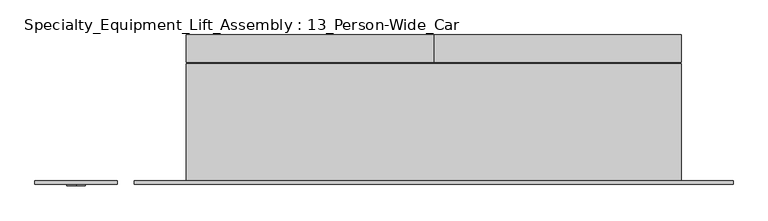
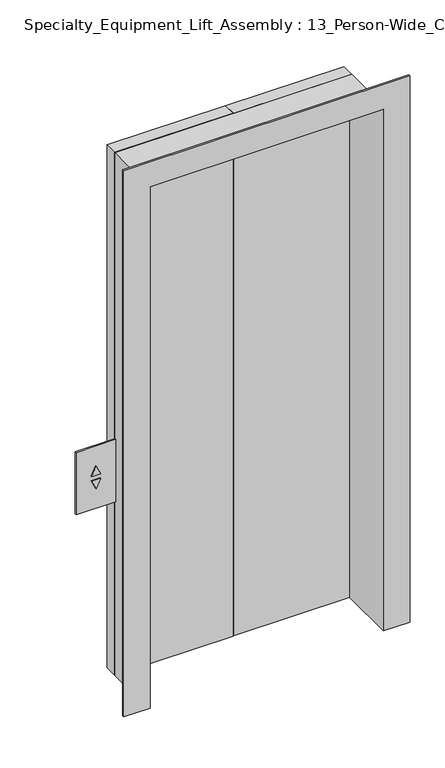
"""IFC4 building model written with IfcOpenShell, lengths in millimetres: proxy geometry, Specialty_Equipment_Lift_Assembly : 13_Person-Wide_Car."""

from ifc_helpers import new_model, si_unit, frame, origin, origin_with_axes, place, context, project, spatial, polyline, outline, extrude, faceted_brep, source, transform, mapped, element, save


def specialty_equipment_lift_assembly_13_person_wide_car_b1ef294d(model_context):
    return source(origin(), model_context, "Body", "SolidModel", [
        extrude(outline(polyline([(1008.7476885, -883.0952695), (1045.0, -900.0), (1008.7476885, -916.9047305), (1008.7476885, -883.0952695)])), frame((0.0, -116.5, 0.0), z_axis=(0.0, 1.0, 0.0), x_axis=(0.0, 0.0, 1.0)), (0.0, 0.0, 1.0), 9.0),
        extrude(outline(polyline([(991.2523115, -883.0952695), (991.2523115, -916.9047305), (955.0, -900.0), (991.2523115, -883.0952695)])), frame((0.0, -116.5, 0.0), z_axis=(0.0, 1.0, 0.0), x_axis=(0.0, 0.0, 1.0)), (0.0, 0.0, 1.0), 9.0),
        extrude(outline(polyline([(200.0, 157.5), (200.0, 107.5), (-249.0, 107.5), (-249.0, 157.5), (200.0, 157.5)])), origin_with_axes(), (0.0, 0.0, 1.0), 2100.0),
        extrude(outline(polyline([(-250.0, 157.5), (-250.0, 107.5), (-700.0, 107.5), (-700.0, 157.5), (-250.0, 157.5)])), origin_with_axes(), (0.0, 0.0, 1.0), 2100.0),
        extrude(outline(polyline([(875.0, -975.0), (875.0, -825.0), (1125.0, -825.0), (1125.0, -975.0), (875.0, -975.0)]), holes=[polyline([(1008.7476885, -883.0952695), (1008.7476885, -916.9047305), (1045.0, -900.0), (1008.7476885, -883.0952695)]), polyline([(991.2523115, -883.0952695), (955.0, -900.0), (991.2523115, -916.9047305), (991.2523115, -883.0952695)])]), frame((0.0, -113.5, 0.0), z_axis=(0.0, 1.0, 0.0), x_axis=(0.0, 0.0, 1.0)), (0.0, 0.0, 1.0), 6.0),
        faceted_brep([(294.0, -113.5, 0.0), (194.0, -113.5, 0.0), (194.0, 105.5, 0.0), (200.0, 105.5, 0.0), (200.0, -107.5, 0.0), (294.0, -107.5, 0.0), (294.0, -107.5, 2194.0), (294.0, -113.5, 2194.0), (200.0, -107.5, 2100.0), (-700.0, -107.5, 2100.0), (-700.0, -107.5, 0.0), (-794.0, -107.5, 0.0), (-794.0, -107.5, 2194.0), (200.0, 105.5, 2100.0), (194.0, 105.5, 2094.0), (-694.0, 105.5, 2094.0), (-694.0, 105.5, 0.0), (-700.0, 105.5, 0.0), (-700.0, 105.5, 2100.0), (194.0, -113.5, 2094.0), (-794.0, -113.5, 2194.0), (-794.0, -113.5, 0.0), (-694.0, -113.5, 0.0), (-694.0, -113.5, 2094.0)], [[[0, 1, 2, 3, 4, 5]], [[5, 6, 7, 0]], [[4, 8, 9, 10, 11, 12, 6, 5]], [[3, 13, 8, 4]], [[2, 14, 15, 16, 17, 18, 13, 3]], [[1, 19, 14, 2]], [[0, 7, 20, 21, 22, 23, 19, 1]], [[6, 12, 20, 7]], [[13, 18, 9, 8]], [[19, 23, 15, 14]], [[21, 11, 10, 17, 16, 22]], [[12, 11, 21, 20]], [[18, 17, 10, 9]], [[23, 22, 16, 15]]]),
    ])


if __name__ == "__main__":
    model = new_model("IFC4")
    model_context = context("Model", 3, world=origin())
    ifc_project = project(units=[si_unit("LENGTHUNIT", "METRE", prefix="MILLI")], contexts=[model_context])
    site = spatial("IfcSite", under=ifc_project)
    building = spatial("IfcBuilding", under=site)
    placement = place(None, origin())
    specialty_equipment_lift_assembly_13_person_wide_car_shape = specialty_equipment_lift_assembly_13_person_wide_car_b1ef294d(model_context)
    element("IfcBuildingElementProxy", 1, Name="Specialty_Equipment_Lift_Assembly : 13_Person-Wide_Car", ObjectType="Specialty_Equipment_Lift_Assembly : 13_Person-Wide_Car", at=placement, inside=building, context=model_context, shape_type="MappedRepresentation", body=[
        mapped(specialty_equipment_lift_assembly_13_person_wide_car_shape, transform((0.0, 0.0, 0.0), x_axis=(1.0, 0.0, 0.0), y_axis=(0.0, 1.0, 0.0), z_axis=(0.0, 0.0, 1.0))),
    ])
    save(model, "model.ifc")

# Revit data of these elements
# Type "Specialty_Equipment_Lift_Assembly : 13_Person-Wide_Car"
#   Keynote = "X"
#   Hoistway Width = 2400 mm
#   Hoistway Depth = 1800 mm
#   Height = 2100 mm
#   Frame Width = 75 mm
#   Percentage Opened (Plan) = 0 mm
#   Door Width = 900 mm
#   Door Trim Width = 100 mm
#   Door Thickness = 50 mm
#   Car Width = 1600 mm
#   Car Thickness = 25 mm
#   Car Front Offset = 250 mm
#   Car Depth = 1400 mm
#   Call Point Z Offset = 1000 mm
#   Call Point X Offset = 200 mm
#   Call Point Panel Width = 150 mm
#   Call Point Panel Depth = 250 mm
#   Vis - Hoistway Location Lines = yes
#   Vis - Door Trim = yes
#   Vis - Call Point = yes
#   Material Trim = Metal - Stainless Steel
#   Material Doors = Metal - Aluminium
#   Wall Closure = (empty or 0)
# Element 1 (IfcBuildingElementProxy, "Specialty_Equipment_Lift_Assembly : 13_Person-Wide_Car")
#   Materials on its faces: "Metal - Stainless Steel", "Metal - Aluminium"
# Materials
#   "Metal - Stainless Steel": class "Metal", colour RGB 252 241 251, transparency 0
#   "Metal - Aluminium": class "Metal", colour RGB 247 247 247, transparency 0
